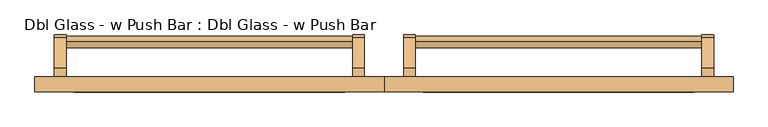
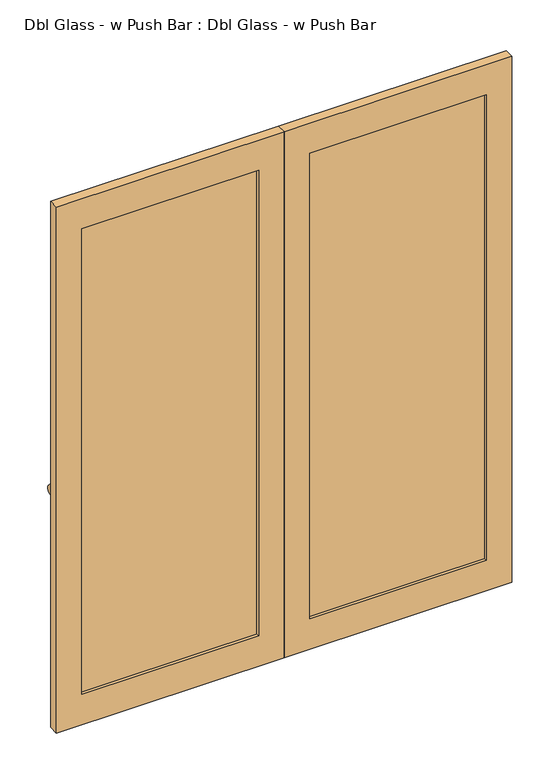
"""IFC4 building model written with IfcOpenShell, lengths in millimetres: door geometry, Dbl Glass - w Push Bar : Dbl Glass - w Push Bar."""

import ifcopenshell
import ifcopenshell.guid

model = None  # the IFC model being written
_history = None  # IfcOwnerHistory: only IFC2X3 demands one
_inside = {}  # id of a spatial element -> (the spatial element, [elements in it])
_under = {}  # id of a project, library or spatial element -> (it, [spatial elements below it])
_declared = {}  # id of a project -> (the project, [libraries it declares])
_typed = {}  # id of a type object -> (the type object, [elements of that type])
_made_of = {}  # id of a material, layer set ... -> (it, [elements and type objects made of it])


def new_model(schema):
    """Start an empty IFC model of exactly this schema.

    Asked for "IFC4X3", IfcOpenShell would pick the latest addendum, in which some entities
    have other attributes; the version numbers below select the first issue.
    IFC2X3 requires an IfcOwnerHistory on every rooted entity: one is made here for all.
    """
    global model, _history
    if schema == "IFC4X3":
        model = ifcopenshell.file(schema_version=(4, 3, 0, 0))
    else:
        model = ifcopenshell.file(schema=schema)
    _inside.clear()
    _under.clear()
    _declared.clear()
    _typed.clear()
    _made_of.clear()
    _history = None
    if model.schema == "IFC2X3":
        org = make("IfcOrganization", Name="unknown")
        user = make(
            "IfcPersonAndOrganization",
            ThePerson=make("IfcPerson", FamilyName="unknown"),
            TheOrganization=org,
        )
        app = make(
            "IfcApplication",
            ApplicationDeveloper=org,
            Version="unknown",
            ApplicationFullName="unknown",
            ApplicationIdentifier="unknown",
        )
        _history = make(
            "IfcOwnerHistory",
            OwningUser=user,
            OwningApplication=app,
            ChangeAction="ADDED",
            CreationDate=0,
        )
    return model


def make(cls, **values):
    """One entity of the class cls with the attributes given. An attribute that is None is left unset."""
    return model.create_entity(
        cls, **{name: value for name, value in values.items() if value is not None}
    )


def rooted(cls, **values):
    """An entity with a GlobalId (a new one), such as an element, a storey or a relation."""
    return make(cls, GlobalId=ifcopenshell.guid.new(), OwnerHistory=_history, **values)


def si_unit(unit_type, name, prefix=None):
    """IfcSIUnit, for example si_unit("LENGTHUNIT", "METRE", prefix="MILLI")."""
    return make("IfcSIUnit", UnitType=unit_type, Prefix=prefix, Name=name)


def assignment(units):
    """IfcUnitAssignment: the units of a project."""
    return None if units is None else make("IfcUnitAssignment", Units=units)


def point(xyz):
    """IfcCartesianPoint."""
    return None if xyz is None else make("IfcCartesianPoint", Coordinates=xyz)


def direction(xyz):
    """IfcDirection."""
    return None if xyz is None else make("IfcDirection", DirectionRatios=xyz)


def frame(location, z_axis=None, x_axis=None):
    """IfcAxis2Placement3D, a coordinate frame: its origin and axes. An axis left out is left unset."""
    return make(
        "IfcAxis2Placement3D",
        Location=point(location),
        Axis=direction(z_axis),
        RefDirection=direction(x_axis),
    )


def frame_2d(location, x_axis=None):
    """IfcAxis2Placement2D, a coordinate frame in the plane: its origin and x axis."""
    return make(
        "IfcAxis2Placement2D", Location=point(location), RefDirection=direction(x_axis)
    )


def origin():
    """The frame at (0, 0, 0) with its axes left unset."""
    return frame((0.0, 0.0, 0.0))


def place(relative_to, where):
    """IfcLocalPlacement: puts the frame where relative to a parent placement (None: the world)."""
    return make(
        "IfcLocalPlacement", PlacementRelTo=relative_to, RelativePlacement=where
    )


def context(
    kind, dimensions, precision=None, world=None, true_north=None, identifier=None
):
    """IfcGeometricRepresentationContext, for example the 3D "Model" context."""
    return make(
        "IfcGeometricRepresentationContext",
        ContextIdentifier=identifier,
        ContextType=kind,
        CoordinateSpaceDimension=dimensions,
        Precision=precision,
        WorldCoordinateSystem=world,
        TrueNorth=true_north,
    )


def project(units=None, contexts=None):
    """IfcProject with its units and contexts."""
    return rooted(
        "IfcProject",
        Name="project",
        RepresentationContexts=contexts,
        UnitsInContext=assignment(units),
    )


def spatial(cls, under=None, at=None, **own):
    """A site, building, storey or space (cls), placed at a placement, below another one or the project."""
    s = rooted(cls, ObjectPlacement=at, **own)
    if under is not None:
        _under.setdefault(under.id(), (under, []))[1].append(s)
    return s


def polyline(points):
    """IfcPolyline through the points."""
    return make("IfcPolyline", Points=[point(p) for p in points])


def circle_curve(where, radius):
    """IfcCircle in the frame where."""
    return make("IfcCircle", Position=where, Radius=radius)


def trimmed(basis, trim1, trim2, sense, master):
    """IfcTrimmedCurve: the piece of a basis curve between two trims."""
    return make(
        "IfcTrimmedCurve",
        BasisCurve=basis,
        Trim1=trim1,
        Trim2=trim2,
        SenseAgreement=sense,
        MasterRepresentation=master,
    )


def segment(curve, same_sense, transition):
    """IfcCompositeCurveSegment."""
    return make(
        "IfcCompositeCurveSegment",
        Transition=transition,
        SameSense=same_sense,
        ParentCurve=curve,
    )


def composite_curve(segments, self_intersect=None):
    """IfcCompositeCurve: segments joined end to end."""
    return make("IfcCompositeCurve", Segments=segments, SelfIntersect=self_intersect)


def outline(outer, holes=None, kind="AREA"):
    """IfcArbitraryClosedProfileDef: a profile drawn as a closed curve; with holes, ...WithVoids."""
    if holes is None:
        return make("IfcArbitraryClosedProfileDef", ProfileType=kind, OuterCurve=outer)
    return make(
        "IfcArbitraryProfileDefWithVoids",
        ProfileType=kind,
        OuterCurve=outer,
        InnerCurves=holes,
    )


def extrude(swept, where, along, depth):
    """IfcExtrudedAreaSolid: the profile swept, set in the frame where, extruded along a direction by depth."""
    return make(
        "IfcExtrudedAreaSolid",
        SweptArea=swept,
        Position=where,
        ExtrudedDirection=direction(along),
        Depth=depth,
    )


def shape(context_of_items, identifier, shape_type, items):
    """IfcShapeRepresentation: the items that make up one representation, for example the "Body"."""
    return make(
        "IfcShapeRepresentation",
        ContextOfItems=context_of_items,
        RepresentationIdentifier=identifier,
        RepresentationType=shape_type,
        Items=items,
    )


def source(mapping_origin, context_of_items, identifier, shape_type, items):
    """IfcRepresentationMap: a shape defined once, which mapped items show again and again."""
    return make(
        "IfcRepresentationMap",
        MappingOrigin=mapping_origin,
        MappedRepresentation=shape(context_of_items, identifier, shape_type, items),
    )


def transform(
    local_origin,
    x_axis=None,
    y_axis=None,
    z_axis=None,
    scale=None,
    scale2=None,
    scale3=None,
    uniform=True,
):
    """IfcCartesianTransformationOperator3D, or its non-uniform kind. x_axis, y_axis, z_axis: its Axis1, 2, 3."""
    if uniform:
        return make(
            "IfcCartesianTransformationOperator3D",
            Axis1=direction(x_axis),
            Axis2=direction(y_axis),
            LocalOrigin=point(local_origin),
            Scale=scale,
            Axis3=direction(z_axis),
        )
    return make(
        "IfcCartesianTransformationOperator3DnonUniform",
        Axis1=direction(x_axis),
        Axis2=direction(y_axis),
        LocalOrigin=point(local_origin),
        Scale=scale,
        Axis3=direction(z_axis),
        Scale2=scale2,
        Scale3=scale3,
    )


def mapped(mapping_source, mapping_target):
    """IfcMappedItem: shows the shape of a source again, moved by a transform."""
    return make(
        "IfcMappedItem", MappingSource=mapping_source, MappingTarget=mapping_target
    )


def made_of(thing, what):
    """Note that an element or type object is made of a material, layer set ...; save() writes the relation."""
    if what is not None:
        _made_of.setdefault(what.id(), (what, []))[1].append(thing)
    return thing


def element(
    cls,
    number,
    at=None,
    inside=None,
    cuts=None,
    type_object=None,
    material=None,
    context=None,
    identifier="Body",
    shape_type=None,
    held_by="IfcProductDefinitionShape",
    body=None,
    shapes=None,
    **own,
):
    """One element of the class cls, such as IfcWall. Its Tag is "e" and its number.

    at: its placement. inside: the storey or other place that contains it. cuts: it is an
    opening in that element (IfcRelVoidsElement). A single representation is given by context,
    identifier, shape_type and body (its items); several are given by shapes. held_by: the class
    of the entity that holds the representations. save() writes the other relations.
    """
    e = rooted(cls, Tag="e%d" % number, ObjectPlacement=at, **own)
    if body is not None:
        shapes = [shape(context, identifier, shape_type, body)]
    if shapes is not None:
        e.Representation = make(held_by, Representations=shapes)
    if inside is not None:
        _inside.setdefault(inside.id(), (inside, []))[1].append(e)
    if cuts is not None:
        rooted(
            "IfcRelVoidsElement", RelatingBuildingElement=cuts, RelatedOpeningElement=e
        )
    if type_object is not None:
        _typed.setdefault(type_object.id(), (type_object, []))[1].append(e)
    return made_of(e, material)


def aggregate(whole, parts):
    """IfcRelAggregates: a whole, such as a stair, and the parts it consists of."""
    return rooted("IfcRelAggregates", RelatingObject=whole, RelatedObjects=parts)


def save(model, path):
    """Write the relations noted so far, then the file.

    IfcRelAggregates (storeys below a building ...), IfcRelContainedInSpatialStructure (elements
    in a storey), IfcRelDefinesByType, IfcRelAssociatesMaterial and IfcRelDeclares: one each for
    every whole, place, type object, material and project.
    """
    for whole, parts in _under.values():
        aggregate(whole, parts)
    for where, things in _inside.values():
        rooted(
            "IfcRelContainedInSpatialStructure",
            RelatedElements=things,
            RelatingStructure=where,
        )
    for kind, things in _typed.values():
        rooted("IfcRelDefinesByType", RelatedObjects=things, RelatingType=kind)
    for what, things in _made_of.values():
        rooted("IfcRelAssociatesMaterial", RelatedObjects=things, RelatingMaterial=what)
    for by, libraries in _declared.values():
        rooted("IfcRelDeclares", RelatingContext=by, RelatedDefinitions=libraries)
    model.write(path)


def dbl_glass_w_push_bar_dbl_glass_w_push_bar_f1c4d891(model_context):
    return source(origin(), model_context, "Body", "SweptSolid", [
        extrude(outline(composite_curve([segment(trimmed(circle_curve(frame_2d((65.0203019, 909.5721086)), 15.0), [point((65.0203019, 924.5721086))], [point((65.0203019, 894.5721086))], False, "CARTESIAN"), True, "CONTINUOUS"), segment(trimmed(circle_curve(frame_2d((65.0203019, 909.5721086)), 15.0), [point((65.0203019, 894.5721086))], [point((65.0203019, 924.5721086))], False, "CARTESIAN"), True, "CONTINUOUS")], self_intersect=False)), frame((80.0, 0.0, 0.0), z_axis=(1.0, 0.0, 0.0), x_axis=(0.0, 1.0, 0.0)), (0.0, 0.0, 1.0), 731.0),
        extrude(outline(composite_curve([segment(polyline([(-0.1563269, 1000.0), (77.6459332, 922.19774)]), True, "CONTINUOUS"), segment(trimmed(circle_curve(frame_2d((65.0203019, 909.5721086)), 17.8553391), [point((77.6459332, 922.19774))], [point((52.3946705, 896.9464773))], False, "CARTESIAN"), True, "CONTINUOUS"), segment(polyline([(52.3946705, 896.9464773), (14.3411478, 935.0), (-24.035259, 935.0), (-24.035259, 1000.0), (-0.1563269, 1000.0)]), True, "CONTINUOUS")], self_intersect=False)), frame((811.0, 0.0, 0.0), z_axis=(1.0, 0.0, 0.0), x_axis=(0.0, 1.0, 0.0)), (0.0, 0.0, 1.0), 30.0),
        extrude(outline(composite_curve([segment(polyline([(-0.1563269, 1000.0), (77.6459332, 922.19774)]), True, "CONTINUOUS"), segment(trimmed(circle_curve(frame_2d((65.0203019, 909.5721086)), 17.8553391), [point((77.6459332, 922.19774))], [point((52.3946705, 896.9464773))], False, "CARTESIAN"), True, "CONTINUOUS"), segment(polyline([(52.3946705, 896.9464773), (14.3411478, 935.0), (-24.035259, 935.0), (-24.035259, 1000.0), (-0.1563269, 1000.0)]), True, "CONTINUOUS")], self_intersect=False)), frame((50.0, 0.0, 0.0), z_axis=(1.0, 0.0, 0.0), x_axis=(0.0, 1.0, 0.0)), (0.0, 0.0, 1.0), 30.0),
        extrude(outline(composite_curve([segment(trimmed(circle_curve(frame_2d((65.0203019, 909.5721086)), 15.0), [point((65.0203019, 924.5721086))], [point((65.0203019, 894.5721086))], False, "CARTESIAN"), True, "CONTINUOUS"), segment(trimmed(circle_curve(frame_2d((65.0203019, 909.5721086)), 15.0), [point((65.0203019, 894.5721086))], [point((65.0203019, 924.5721086))], False, "CARTESIAN"), True, "CONTINUOUS")], self_intersect=False)), frame((-811.0, 0.0, 0.0), z_axis=(1.0, 0.0, 0.0), x_axis=(0.0, 1.0, 0.0)), (0.0, 0.0, 1.0), 731.0),
        extrude(outline(composite_curve([segment(polyline([(-0.1563269, 1000.0), (77.6459332, 922.19774)]), True, "CONTINUOUS"), segment(trimmed(circle_curve(frame_2d((65.0203019, 909.5721086)), 17.8553391), [point((77.6459332, 922.19774))], [point((52.3946705, 896.9464773))], False, "CARTESIAN"), True, "CONTINUOUS"), segment(polyline([(52.3946705, 896.9464773), (14.3411478, 935.0), (-24.035259, 935.0), (-24.035259, 1000.0), (-0.1563269, 1000.0)]), True, "CONTINUOUS")], self_intersect=False)), frame((-80.0, 0.0, 0.0), z_axis=(1.0, 0.0, 0.0), x_axis=(0.0, 1.0, 0.0)), (0.0, 0.0, 1.0), 30.0),
        extrude(outline(composite_curve([segment(polyline([(-0.1563269, 1000.0), (77.6459332, 922.19774)]), True, "CONTINUOUS"), segment(trimmed(circle_curve(frame_2d((65.0203019, 909.5721086)), 17.8553391), [point((77.6459332, 922.19774))], [point((52.3946705, 896.9464773))], False, "CARTESIAN"), True, "CONTINUOUS"), segment(polyline([(52.3946705, 896.9464773), (14.3411478, 935.0), (-24.035259, 935.0), (-24.035259, 1000.0), (-0.1563269, 1000.0)]), True, "CONTINUOUS")], self_intersect=False)), frame((-841.0, 0.0, 0.0), z_axis=(1.0, 0.0, 0.0), x_axis=(0.0, 1.0, 0.0)), (0.0, 0.0, 1.0), 30.0),
        extrude(outline(polyline([(2175.0, -891.0), (0.0, -891.0), (0.0, 0.0), (2175.0, 0.0), (2175.0, -891.0)]), holes=[polyline([(2050.0, -791.0), (2050.0, -100.0), (125.0, -100.0), (125.0, -791.0), (2050.0, -791.0)])]), frame((0.0, -62.5788556, 0.0), z_axis=(0.0, 1.0, 0.0), x_axis=(0.0, 0.0, 1.0)), (0.0, 0.0, 1.0), 38.5435966),
        extrude(outline(polyline([(2175.0, 0.0), (0.0, 0.0), (0.0, 891.0), (2175.0, 891.0), (2175.0, 0.0)]), holes=[polyline([(2050.0, 100.0), (2050.0, 791.0), (125.0, 791.0), (125.0, 100.0), (2050.0, 100.0)])]), frame((0.0, -62.5788556, 0.0), z_axis=(0.0, 1.0, 0.0), x_axis=(0.0, 0.0, 1.0)), (0.0, 0.0, 1.0), 38.5435966),
        extrude(outline(polyline([(-100.0, -38.0), (-100.0, -50.0), (-791.0, -50.0), (-791.0, -38.0), (-100.0, -38.0)])), frame((0.0, 0.0, 125.0), z_axis=(0.0, 0.0, 1.0), x_axis=(1.0, 0.0, 0.0)), (0.0, 0.0, 1.0), 1925.0),
        extrude(outline(polyline([(791.0, -38.0), (791.0, -50.0), (100.0, -50.0), (100.0, -38.0), (791.0, -38.0)])), frame((0.0, 0.0, 125.0), z_axis=(0.0, 0.0, 1.0), x_axis=(1.0, 0.0, 0.0)), (0.0, 0.0, 1.0), 1925.0),
    ])


if __name__ == "__main__":
    model = new_model("IFC4")
    model_context = context("Model", 3, world=origin())
    ifc_project = project(units=[si_unit("LENGTHUNIT", "METRE", prefix="MILLI")], contexts=[model_context])
    site = spatial("IfcSite", under=ifc_project)
    building = spatial("IfcBuilding", under=site)
    placement = place(None, origin())
    dbl_glass_w_push_bar_dbl_glass_w_push_bar_shape = dbl_glass_w_push_bar_dbl_glass_w_push_bar_f1c4d891(model_context)
    element("IfcDoor", 1, ObjectType="Dbl Glass - w Push Bar : Dbl Glass - w Push Bar", at=placement, inside=building, context=model_context, shape_type="MappedRepresentation", body=[
        mapped(dbl_glass_w_push_bar_dbl_glass_w_push_bar_shape, transform((0.0, 0.0, 0.0), x_axis=(1.0, 0.0, 0.0), y_axis=(0.0, 1.0, 0.0), z_axis=(0.0, 0.0, 1.0))),
    ])
    save(model, "model.ifc")

# Revit data of these elements
# Type "Dbl Glass - w Push Bar : Dbl Glass - w Push Bar"
#   Description = "Curtain Wall Door"
#   Type Mark = "55"
#   Construction Type Id = "GSP4R"
#   Analytic Construction = "1/8 in Pilkington single glazing"
#   Visual Light Transmittance = 0.9
#   TopRail = 125 mm
#   Solar Heat Gain Coefficient = 0.78
#   Offset = 50 mm
#   MuntinRail = 100 mm
#   LockRail = 100 mm
#   Heat Transfer Coefficient (U) = 3.6886 W/(m²·K)
#   Handle Z Distance = 1000 mm
#   Handle X Offset = 65 mm
#   Glass Thickness = 12 mm
#   BottomRail = 125 mm
#   Define Thermal Properties by = 1
#   Material Ironmongery = Metal - Aluminum
#   Material Door = Metal - Aluminum
#   Material Glass = Glass
#   Function = (empty or 0)
# Element 1 (IfcDoor, "Dbl Glass - w Push Bar : Dbl Glass - w Push Bar")
#   Materials on its faces: "Metal - Aluminum", "Glass"
# Materials
#   "Metal - Aluminum": class "Metal", colour RGB 247 247 247, transparency 0
#   "Glass": class "Glass", colour RGB 0 128 192, transparency 0.9, Description = "Soda Lime Glass", Cost = 0
